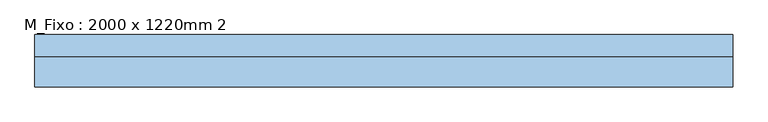
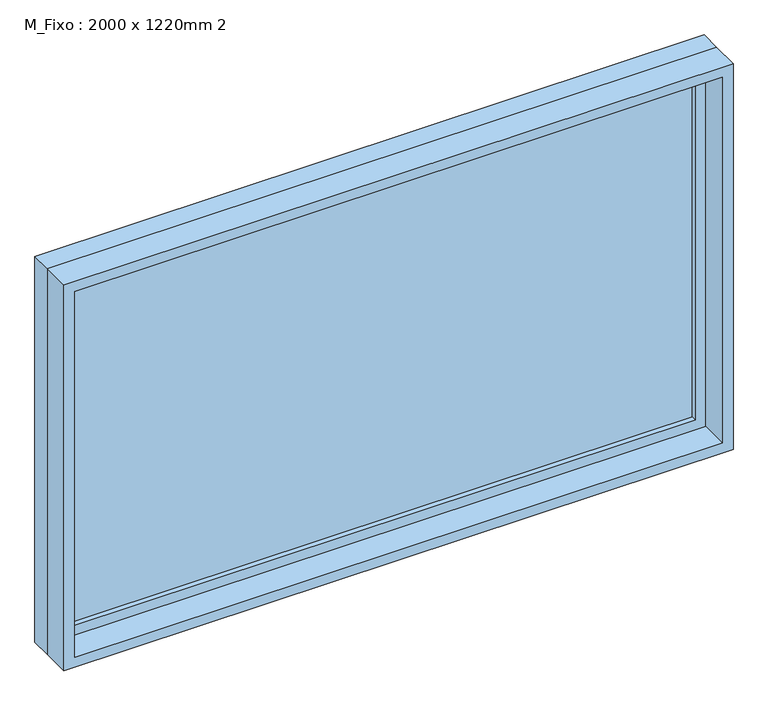
"""IFC4 building model written with IfcOpenShell, lengths in millimetres: window geometry, M_Fixo : 2000 x 1220mm 2."""

from ifc_helpers import new_model, si_unit, frame, origin, place, context, project, spatial, polyline, outline, extrude, source, transform, mapped, element, save


def m_fixo_2000_x_1220mm_2_8e554ddc(model_context):
    return source(origin(), model_context, "Body", "SweptSolid", [
        extrude(outline(polyline([(-937.0, 53.0), (937.0, 53.0), (937.0, 41.0), (-937.0, 41.0), (-937.0, 53.0)])), frame((0.0, 0.0, 978.0), z_axis=(0.0, 0.0, 1.0), x_axis=(1.0, 0.0, 0.0)), (0.0, 0.0, 1.0), 1094.0),
        extrude(outline(polyline([(2116.0, -981.0), (934.0, -981.0), (934.0, 981.0), (2116.0, 981.0), (2116.0, -981.0)]), holes=[polyline([(2072.0, -937.0), (2072.0, 937.0), (978.0, 937.0), (978.0, -937.0), (2072.0, -937.0)])]), frame((0.0, 25.0, 0.0), z_axis=(0.0, 1.0, 0.0), x_axis=(0.0, 0.0, 1.0)), (0.0, 0.0, 1.0), 44.0),
        extrude(outline(polyline([(2135.0, -1000.0), (915.0, -1000.0), (915.0, 1000.0), (2135.0, 1000.0), (2135.0, -1000.0)]), holes=[polyline([(2116.0, -981.0), (2116.0, 981.0), (934.0, 981.0), (934.0, -981.0), (2116.0, -981.0)])]), frame((0.0, 25.0, 0.0), z_axis=(0.0, 1.0, 0.0), x_axis=(0.0, 0.0, 1.0)), (0.0, 0.0, 1.0), 63.0),
        extrude(outline(polyline([(2135.0, -1000.0), (915.0, -1000.0), (915.0, 1000.0), (2135.0, 1000.0), (2135.0, -1000.0)]), holes=[polyline([(2103.0, -968.0), (2103.0, 968.0), (947.0, 968.0), (947.0, -968.0), (2103.0, -968.0)])]), frame((0.0, -62.0, 0.0), z_axis=(0.0, 1.0, 0.0), x_axis=(0.0, 0.0, 1.0)), (0.0, 0.0, 1.0), 87.0),
    ])


if __name__ == "__main__":
    model = new_model("IFC4")
    model_context = context("Model", 3, world=origin())
    ifc_project = project(units=[si_unit("LENGTHUNIT", "METRE", prefix="MILLI")], contexts=[model_context])
    site = spatial("IfcSite", under=ifc_project)
    building = spatial("IfcBuilding", under=site)
    placement = place(None, origin())
    m_fixo_2000_x_1220mm_2_shape = m_fixo_2000_x_1220mm_2_8e554ddc(model_context)
    element("IfcWindow", 1, ObjectType="M_Fixo : 2000 x 1220mm 2", at=placement, inside=building, context=model_context, shape_type="MappedRepresentation", body=[
        mapped(m_fixo_2000_x_1220mm_2_shape, transform((0.0, 0.0, 0.0), x_axis=(1.0, 0.0, 0.0), y_axis=(0.0, 1.0, 0.0), z_axis=(0.0, 0.0, 1.0))),
    ])
    save(model, "model.ifc")

# Revit data of these elements
# Type "M_Fixo : 2000 x 1220mm 2"
#   Type Mark = "19"
#   Construction Type Id = "GSP4R"
#   Analytic Construction = "Vidraça única Pilkington 1/8 pol"
#   Visual Light Transmittance = 0.9
#   Thermal Resistance (R) = 0.271106 (m²·K)/W
#   Solar Heat Gain Coefficient = 0.78
#   Heat Transfer Coefficient (U) = 3.6886 W/(m²·K)
#   Height = 1.22 m
#   Altura-padrão do peitoril = 0.915 m
#   Width = 2.00 m
#   Janela aplicada = 0.019 m
#   Material da estrutura externa = Caixilho
#   Material da estrutura interna = Caixilho
#   Material do painel de vidro = Vidro
#   Caixilho = Caixilho
#   Wall Closure = (empty or 0)
# Element 1 (IfcWindow, "M_Fixo : 2000 x 1220mm 2")
#   Materials on its faces: "Caixilho", "Vidro"
# Materials
#   "Caixilho": class "Madeira", colour RGB 224 178 126, transparency 0, Cost = 0
#   "Vidro": class "Vidro", colour RGB 0 128 192, transparency 0.9, Description = "Vidro de sílica", Cost = 0
